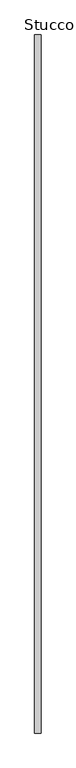
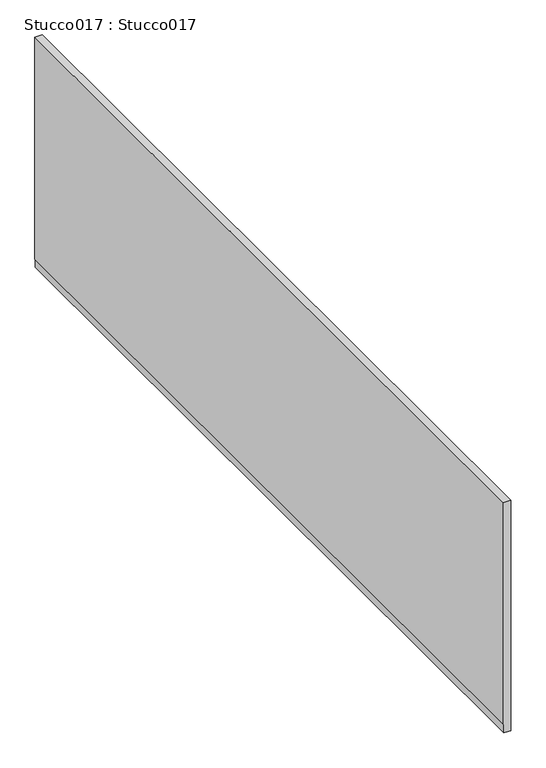
"""IFC4 building model written with IfcOpenShell, lengths in millimetres: proxy geometry, Stucco017 : Stucco017."""

from ifc_helpers import new_model, si_unit, frame, origin, place, context, project, spatial, polyline, outline, extrude, source, transform, mapped, element, save


def stucco017_stucco017_1e404a43(model_context):
    return source(origin(), model_context, "Body", "SweptSolid", [
        extrude(outline(polyline([(39567.688258, -7249.6322073), (39567.688258, -7248.347187), (39545.1576447, -7248.347187), (39545.1576447, -7231.8520027), (40145.4616445, -7231.8520027), (40145.4616445, -7249.6322073), (39567.688258, -7249.6322073)])), frame((0.0, 7982.1532461, 0.0), z_axis=(0.0, 1.0, 0.0), x_axis=(0.0, 0.0, 1.0)), (0.0, 0.0, 1.0), 1999.9999999),
    ])


if __name__ == "__main__":
    model = new_model("IFC4")
    model_context = context("Model", 3, world=origin())
    ifc_project = project(units=[si_unit("LENGTHUNIT", "METRE", prefix="MILLI")], contexts=[model_context])
    site = spatial("IfcSite", under=ifc_project)
    building = spatial("IfcBuilding", under=site)
    placement = place(None, origin())
    stucco017_stucco017_shape = stucco017_stucco017_1e404a43(model_context)
    element("IfcBuildingElementProxy", 1, Name="Stucco017 : Stucco017", ObjectType="Stucco017 : Stucco017", at=placement, inside=building, context=model_context, shape_type="MappedRepresentation", body=[
        mapped(stucco017_stucco017_shape, transform((0.0, 0.0, 0.0), x_axis=(1.0, 0.0, 0.0), y_axis=(0.0, 1.0, 0.0), z_axis=(0.0, 0.0, 1.0))),
    ])
    save(model, "model.ifc")

# Revit data of these elements
# Type "Stucco017 : Stucco017"
#   NameOverride = "Stucco017"
# Element 1 (IfcBuildingElementProxy, "Stucco017 : Stucco017")
#   Materials on its faces: "7/8\" SMOOTH TROWEL EXTERIOR STUCCO"
# Materials
#   "7/8\" SMOOTH TROWEL EXTERIOR STUCCO": class "Unassigned", colour RGB 255 255 255, transparency 0, Cost = 0
